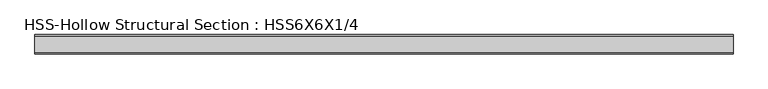
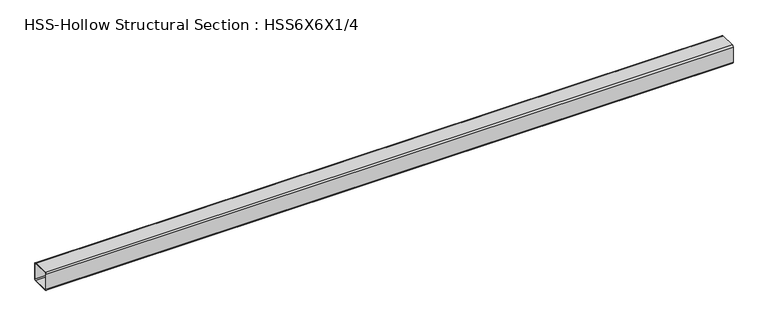
"""IFC4 building model written with IfcOpenShell, lengths in millimetres: beam geometry, HSS-Hollow Structural Section : HSS6X6X1/4."""

from ifc_helpers import new_model, si_unit, point, frame, frame_2d, origin, place, context, project, spatial, polyline, circle_curve, trimmed, segment, composite_curve, outline, extrude, source, transform, mapped, element, save


def hss_hollow_structural_section_hss6x6x1_4_9a0f4812(model_context):
    return source(origin(), model_context, "Body", "SweptSolid", [
        extrude(outline(composite_curve([segment(polyline([(76.2, 64.3636), (76.2, -64.3636)]), True, "CONTINUOUS"), segment(trimmed(circle_curve(frame_2d((64.3636, -64.3636)), 11.8364), [point((76.2, -64.3636))], [point((64.3636, -76.2))], False, "CARTESIAN"), True, "CONTINUOUS"), segment(polyline([(64.3636, -76.2), (-64.3636, -76.2)]), True, "CONTINUOUS"), segment(trimmed(circle_curve(frame_2d((-64.3636, -64.3636)), 11.8364), [point((-64.3636, -76.2))], [point((-76.2, -64.3636))], False, "CARTESIAN"), True, "CONTINUOUS"), segment(polyline([(-76.2, -64.3636), (-76.2, 64.3636)]), True, "CONTINUOUS"), segment(trimmed(circle_curve(frame_2d((-64.3636, 64.3636)), 11.8364), [point((-76.2, 64.3636))], [point((-64.3636, 76.2))], False, "CARTESIAN"), True, "CONTINUOUS"), segment(polyline([(-64.3636, 76.2), (64.3636, 76.2)]), True, "CONTINUOUS"), segment(trimmed(circle_curve(frame_2d((64.3636, 64.3636)), 11.8364), [point((64.3636, 76.2))], [point((76.2, 64.3636))], False, "CARTESIAN"), True, "CONTINUOUS")], self_intersect=False), holes=[composite_curve([segment(trimmed(circle_curve(frame_2d((-64.3636, 64.3636)), 5.9182), [point((-64.3636, 70.2818))], [point((-70.2818, 64.3636))], True, "CARTESIAN"), True, "CONTINUOUS"), segment(polyline([(-70.2818, 64.3636), (-70.2818, -64.3636)]), True, "CONTINUOUS"), segment(trimmed(circle_curve(frame_2d((-64.3636, -64.3636)), 5.9182), [point((-70.2818, -64.3636))], [point((-64.3636, -70.2818))], True, "CARTESIAN"), True, "CONTINUOUS"), segment(polyline([(-64.3636, -70.2818), (64.3636, -70.2818)]), True, "CONTINUOUS"), segment(trimmed(circle_curve(frame_2d((64.3636, -64.3636)), 5.9182), [point((64.3636, -70.2818))], [point((70.2818, -64.3636))], True, "CARTESIAN"), True, "CONTINUOUS"), segment(polyline([(70.2818, -64.3636), (70.2818, 64.3636)]), True, "CONTINUOUS"), segment(trimmed(circle_curve(frame_2d((64.3636, 64.3636)), 5.9182), [point((70.2818, 64.3636))], [point((64.3636, 70.2818))], True, "CARTESIAN"), True, "CONTINUOUS"), segment(polyline([(64.3636, 70.2818), (-64.3636, 70.2818)]), True, "CONTINUOUS")], self_intersect=False)]), frame((-2755.9, 0.0, 0.0), z_axis=(1.0, 0.0, 0.0), x_axis=(0.0, 1.0, 0.0)), (0.0, 0.0, 1.0), 5511.8),
    ])


if __name__ == "__main__":
    model = new_model("IFC4")
    model_context = context("Model", 3, world=origin())
    ifc_project = project(units=[si_unit("LENGTHUNIT", "METRE", prefix="MILLI")], contexts=[model_context])
    site = spatial("IfcSite", under=ifc_project)
    building = spatial("IfcBuilding", under=site)
    placement = place(None, origin())
    hss_hollow_structural_section_hss6x6x1_4_shape = hss_hollow_structural_section_hss6x6x1_4_9a0f4812(model_context)
    element("IfcBeam", 1, ObjectType="HSS-Hollow Structural Section : HSS6X6X1/4", at=placement, inside=building, context=model_context, shape_type="MappedRepresentation", body=[
        mapped(hss_hollow_structural_section_hss6x6x1_4_shape, transform((0.0, 0.0, 0.0), x_axis=(1.0, 0.0, 0.0), y_axis=(0.0, 1.0, 0.0), z_axis=(0.0, 0.0, 1.0))),
    ])
    save(model, "model.ifc")

# Revit data of these elements
# Type "HSS-Hollow Structural Section : HSS6X6X1/4"
#   Assembly Code = "B10"
#   Shape = "Square"
#   W = 19
#   Ht = 0' - 6"
#   Length [instance default] = 5' - 0"
#   b = 0' - 6"
#   kr = 0' - 0.466"
#   t = 0' - 0.233"
#   A = 0.0363889 SF
#   Structural Material [instance default] = Steel ASTM A500, Grade B, Rectangular and Square
# Element 1 (IfcBeam, "HSS-Hollow Structural Section : HSS6X6X1/4")
#   Materials on its faces: "Steel ASTM A500, Grade B, Rectangular and Square"
# Materials
#   "Steel ASTM A500, Grade B, Rectangular and Square": class "Metal", colour RGB 199 199 199, transparency 0, Description = "Carbon steel", Cost = 0
